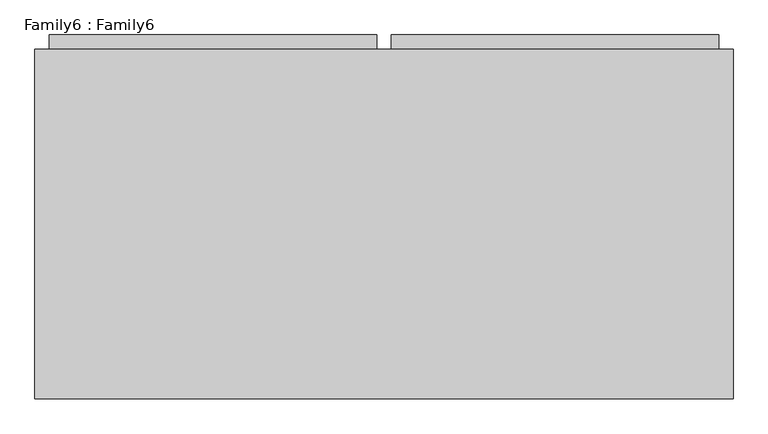
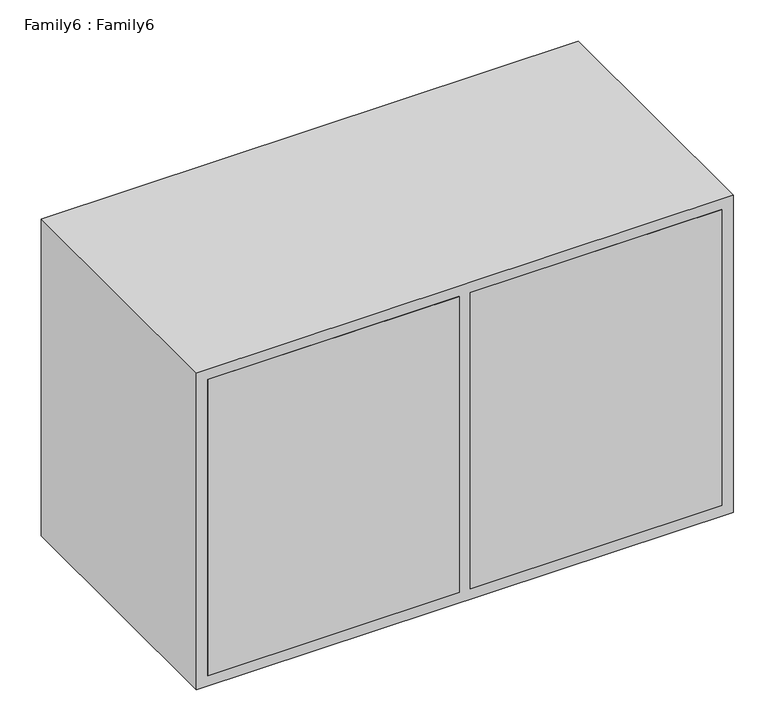
"""IFC4 building model written with IfcOpenShell, lengths in millimetres: proxy geometry, Family6 : Family6."""

from ifc_helpers import new_model, si_unit, frame, origin, place, context, project, spatial, polyline, outline, extrude, source, transform, mapped, element, save


def family6_family6_469ca9a8(model_context):
    return source(origin(), model_context, "Body", "SweptSolid", [
        extrude(outline(polyline([(12.7, 685.8), (584.2, 685.8), (584.2, 50.8), (12.7, 50.8), (12.7, 685.8)])), frame((0.0, 0.0, 1292.514135), z_axis=(0.0, 0.0, 1.0), x_axis=(1.0, 0.0, 0.0)), (0.0, 0.0, 1.0), 711.2),
        extrude(outline(polyline([(-584.2, 685.8), (-12.7, 685.8), (-12.7, 50.8), (-584.2, 50.8), (-584.2, 685.8)])), frame((0.0, 0.0, 1292.514135), z_axis=(0.0, 0.0, 1.0), x_axis=(1.0, 0.0, 0.0)), (0.0, 0.0, 1.0), 711.2),
        extrude(outline(polyline([(-609.6, 660.4), (609.6, 660.4), (609.6, 50.8), (-609.6, 50.8), (-609.6, 660.4)])), frame((0.0, 0.0, 1267.114135), z_axis=(0.0, 0.0, 1.0), x_axis=(1.0, 0.0, 0.0)), (0.0, 0.0, 1.0), 762.0),
    ])


if __name__ == "__main__":
    model = new_model("IFC4")
    model_context = context("Model", 3, world=origin())
    ifc_project = project(units=[si_unit("LENGTHUNIT", "METRE", prefix="MILLI")], contexts=[model_context])
    site = spatial("IfcSite", under=ifc_project)
    building = spatial("IfcBuilding", under=site)
    placement = place(None, origin())
    family6_family6_shape = family6_family6_469ca9a8(model_context)
    element("IfcBuildingElementProxy", 1, Name="Family6 : Family6", ObjectType="Family6 : Family6", at=placement, inside=building, context=model_context, shape_type="MappedRepresentation", body=[
        mapped(family6_family6_shape, transform((0.0, 0.0, 0.0), x_axis=(1.0, 0.0, 0.0), y_axis=(0.0, 1.0, 0.0), z_axis=(0.0, 0.0, 1.0))),
    ])
    save(model, "model.ifc")

# Revit data of these elements
# Type "Family6 : Family6"
#   total width = 4' - 0"
#   middle strip distance = 0' - 1"
#   drawer depth = 2' - 1"
#   cabinet depth = 2' - 0"
#   Default Elevation = 0
